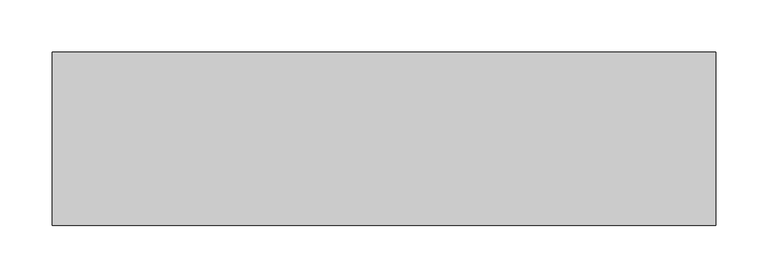
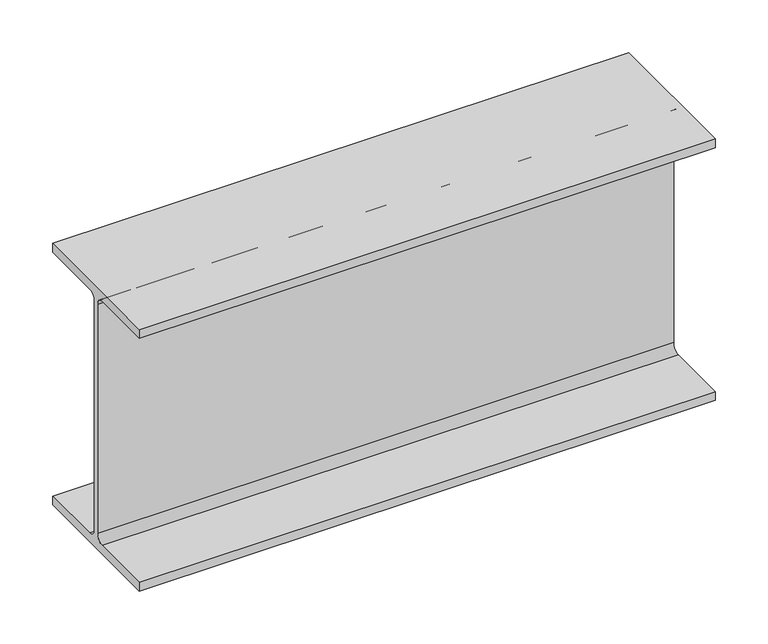
"""IFC4 building model written with IfcOpenShell, lengths in millimetres: beam geometry, Old_Steel Beam_H-KSD3502 : H_SB_ASB_H-300×150x6.5x9."""

from ifc_helpers import new_model, si_unit, point, frame, frame_2d, origin, place, context, project, spatial, polyline, circle_curve, trimmed, segment, composite_curve, outline, extrude, source, transform, mapped, element, save


def beam_96c0519e(model_context):
    return source(origin(), model_context, "Body", "SweptSolid", [
        extrude(outline(composite_curve([segment(polyline([(82.5, -141.5), (82.5, -151.7), (-82.5, -151.7), (-82.5, -141.5), (-11.9, -141.5)]), True, "CONTINUOUS"), segment(trimmed(circle_curve(frame_2d((-11.9, -132.6)), 8.9), [point((-11.9, -141.5))], [point((-3.0, -132.6))], True, "CARTESIAN"), True, "CONTINUOUS"), segment(polyline([(-3.0, -132.6), (-3.0, 132.6)]), True, "CONTINUOUS"), segment(trimmed(circle_curve(frame_2d((-11.9, 132.6)), 8.9), [point((-3.0, 132.6))], [point((-11.9, 141.5))], True, "CARTESIAN"), True, "CONTINUOUS"), segment(polyline([(-11.9, 141.5), (-82.5, 141.5), (-82.5, 151.7), (82.5, 151.7), (82.5, 141.5), (11.9, 141.5)]), True, "CONTINUOUS"), segment(trimmed(circle_curve(frame_2d((11.9, 132.6)), 8.9), [point((11.9, 141.5))], [point((3.0, 132.6))], True, "CARTESIAN"), True, "CONTINUOUS"), segment(polyline([(3.0, 132.6), (3.0, -132.6)]), True, "CONTINUOUS"), segment(trimmed(circle_curve(frame_2d((11.9, -132.6)), 8.9), [point((3.0, -132.6))], [point((11.9, -141.5))], True, "CARTESIAN"), True, "CONTINUOUS"), segment(polyline([(11.9, -141.5), (82.5, -141.5)]), True, "CONTINUOUS")], self_intersect=False)), frame((-238.55, 0.0, 0.0), z_axis=(1.0, 0.0, 0.0), x_axis=(0.0, 1.0, 0.0)), (0.0, 0.0, 1.0), 632.1),
    ])


if __name__ == "__main__":
    model = new_model("IFC4")
    model_context = context("Model", 3, world=origin())
    ifc_project = project(units=[si_unit("LENGTHUNIT", "METRE", prefix="MILLI")], contexts=[model_context])
    site = spatial("IfcSite", under=ifc_project)
    building = spatial("IfcBuilding", under=site)
    placement = place(None, origin())
    beam_shape = beam_96c0519e(model_context)
    element("IfcBeam", 1, ObjectType="Old_Steel Beam_H-KSD3502 : H_SB_ASB_H-300×150x6.5x9", at=placement, inside=building, context=model_context, shape_type="MappedRepresentation", body=[
        mapped(beam_shape, transform((0.0, 0.0, 0.0), x_axis=(1.0, 0.0, 0.0), y_axis=(0.0, 1.0, 0.0), z_axis=(0.0, 0.0, 1.0))),
    ])
    save(model, "model.ifc")

# Revit data of these elements
# Type "Old_Steel Beam_H-KSD3502 : H_SB_ASB_H-300×150x6.5x9"
#   Width = 15.0 cm
#   Web Thickness = 0.65 cm
#   Web Fillet = 1.3 cm
#   Warping Constant = 107174.0 cm⁶
#   Torsional Moment of Inertia = 9.9539 cm⁴
#   Torsional Modulus = 1.0 cm³
#   Section Area = 46.78 cm²
#   Plastic Modulus weak axis = 105.0 cm³
#   Plastic Modulus strong axis = 542.0 cm³
#   Perimeter = 1.17 m²/m
#   Nominal Weight = 36.70 kgf/m
#   Moment of Inertia weak axis = 508.00 cm⁴
#   Moment of Inertia strong axis = 7210.00 cm⁴
#   Height = 30.0 cm
#   Flange Thickness = 0.9 cm
#   Elastic Modulus weak axis = 67.7 cm³
#   Elastic Modulus strong axis = 481.0 cm³
#   Centroid Vertical = 15.0 cm
#   Centroid Horizontal = 7.5 cm
#   Length [instance default] = 1.5240 m
#   Structural Material [instance default] = Steel, 45-345
#   Assembly Code = ""
# Element 1 (IfcBeam, "Old_Steel Beam_H-KSD3502 : H_SB_ASB_H-300×150x6.5x9")
#   Structural Material = none
# Materials
#   "Steel, 45-345": class "Metal", colour RGB 189 187 185, transparency 0, Description = "Steel 345 MPa", Cost = 0
